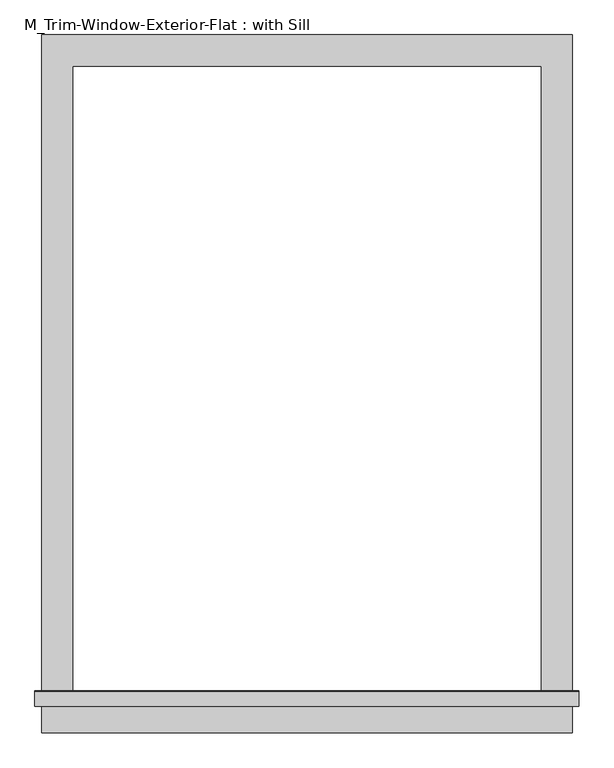
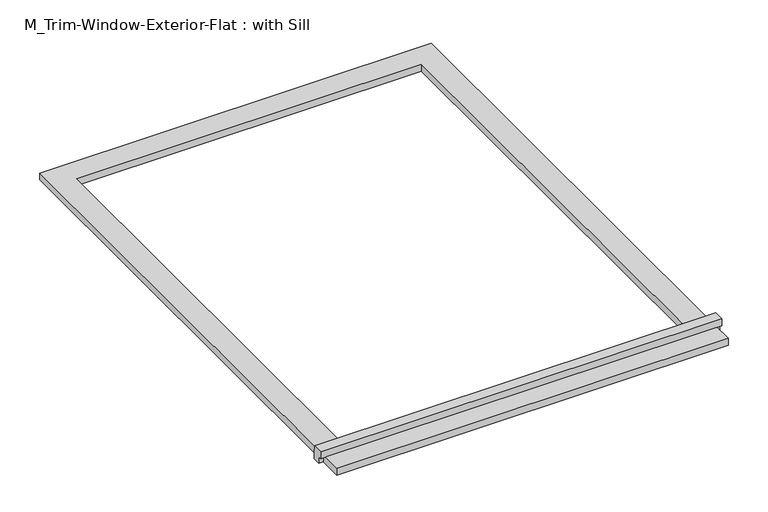
"""IFC4 building model written with IfcOpenShell, lengths in millimetres: proxy geometry, M_Trim-Window-Exterior-Flat : with Sill."""

import ifcopenshell
import ifcopenshell.guid

model = None  # the IFC model being written
_history = None  # IfcOwnerHistory: only IFC2X3 demands one
_inside = {}  # id of a spatial element -> (the spatial element, [elements in it])
_under = {}  # id of a project, library or spatial element -> (it, [spatial elements below it])
_declared = {}  # id of a project -> (the project, [libraries it declares])
_typed = {}  # id of a type object -> (the type object, [elements of that type])
_made_of = {}  # id of a material, layer set ... -> (it, [elements and type objects made of it])


def new_model(schema):
    """Start an empty IFC model of exactly this schema.

    Asked for "IFC4X3", IfcOpenShell would pick the latest addendum, in which some entities
    have other attributes; the version numbers below select the first issue.
    IFC2X3 requires an IfcOwnerHistory on every rooted entity: one is made here for all.
    """
    global model, _history
    if schema == "IFC4X3":
        model = ifcopenshell.file(schema_version=(4, 3, 0, 0))
    else:
        model = ifcopenshell.file(schema=schema)
    _inside.clear()
    _under.clear()
    _declared.clear()
    _typed.clear()
    _made_of.clear()
    _history = None
    if model.schema == "IFC2X3":
        org = make("IfcOrganization", Name="unknown")
        user = make(
            "IfcPersonAndOrganization",
            ThePerson=make("IfcPerson", FamilyName="unknown"),
            TheOrganization=org,
        )
        app = make(
            "IfcApplication",
            ApplicationDeveloper=org,
            Version="unknown",
            ApplicationFullName="unknown",
            ApplicationIdentifier="unknown",
        )
        _history = make(
            "IfcOwnerHistory",
            OwningUser=user,
            OwningApplication=app,
            ChangeAction="ADDED",
            CreationDate=0,
        )
    return model


def make(cls, **values):
    """One entity of the class cls with the attributes given. An attribute that is None is left unset."""
    return model.create_entity(
        cls, **{name: value for name, value in values.items() if value is not None}
    )


def rooted(cls, **values):
    """An entity with a GlobalId (a new one), such as an element, a storey or a relation."""
    return make(cls, GlobalId=ifcopenshell.guid.new(), OwnerHistory=_history, **values)


def si_unit(unit_type, name, prefix=None):
    """IfcSIUnit, for example si_unit("LENGTHUNIT", "METRE", prefix="MILLI")."""
    return make("IfcSIUnit", UnitType=unit_type, Prefix=prefix, Name=name)


def assignment(units):
    """IfcUnitAssignment: the units of a project."""
    return None if units is None else make("IfcUnitAssignment", Units=units)


def point(xyz):
    """IfcCartesianPoint."""
    return None if xyz is None else make("IfcCartesianPoint", Coordinates=xyz)


def direction(xyz):
    """IfcDirection."""
    return None if xyz is None else make("IfcDirection", DirectionRatios=xyz)


def frame(location, z_axis=None, x_axis=None):
    """IfcAxis2Placement3D, a coordinate frame: its origin and axes. An axis left out is left unset."""
    return make(
        "IfcAxis2Placement3D",
        Location=point(location),
        Axis=direction(z_axis),
        RefDirection=direction(x_axis),
    )


def origin():
    """The frame at (0, 0, 0) with its axes left unset."""
    return frame((0.0, 0.0, 0.0))


def origin_with_axes():
    """The frame at (0, 0, 0) with the z axis (0, 0, 1) and the x axis (1, 0, 0) written out."""
    return frame((0.0, 0.0, 0.0), z_axis=(0.0, 0.0, 1.0), x_axis=(1.0, 0.0, 0.0))


def place(relative_to, where):
    """IfcLocalPlacement: puts the frame where relative to a parent placement (None: the world)."""
    return make(
        "IfcLocalPlacement", PlacementRelTo=relative_to, RelativePlacement=where
    )


def context(
    kind, dimensions, precision=None, world=None, true_north=None, identifier=None
):
    """IfcGeometricRepresentationContext, for example the 3D "Model" context."""
    return make(
        "IfcGeometricRepresentationContext",
        ContextIdentifier=identifier,
        ContextType=kind,
        CoordinateSpaceDimension=dimensions,
        Precision=precision,
        WorldCoordinateSystem=world,
        TrueNorth=true_north,
    )


def project(units=None, contexts=None):
    """IfcProject with its units and contexts."""
    return rooted(
        "IfcProject",
        Name="project",
        RepresentationContexts=contexts,
        UnitsInContext=assignment(units),
    )


def spatial(cls, under=None, at=None, **own):
    """A site, building, storey or space (cls), placed at a placement, below another one or the project."""
    s = rooted(cls, ObjectPlacement=at, **own)
    if under is not None:
        _under.setdefault(under.id(), (under, []))[1].append(s)
    return s


def polyline(points):
    """IfcPolyline through the points."""
    return make("IfcPolyline", Points=[point(p) for p in points])


def outline(outer, holes=None, kind="AREA"):
    """IfcArbitraryClosedProfileDef: a profile drawn as a closed curve; with holes, ...WithVoids."""
    if holes is None:
        return make("IfcArbitraryClosedProfileDef", ProfileType=kind, OuterCurve=outer)
    return make(
        "IfcArbitraryProfileDefWithVoids",
        ProfileType=kind,
        OuterCurve=outer,
        InnerCurves=holes,
    )


def extrude(swept, where, along, depth):
    """IfcExtrudedAreaSolid: the profile swept, set in the frame where, extruded along a direction by depth."""
    return make(
        "IfcExtrudedAreaSolid",
        SweptArea=swept,
        Position=where,
        ExtrudedDirection=direction(along),
        Depth=depth,
    )


def shape(context_of_items, identifier, shape_type, items):
    """IfcShapeRepresentation: the items that make up one representation, for example the "Body"."""
    return make(
        "IfcShapeRepresentation",
        ContextOfItems=context_of_items,
        RepresentationIdentifier=identifier,
        RepresentationType=shape_type,
        Items=items,
    )


def source(mapping_origin, context_of_items, identifier, shape_type, items):
    """IfcRepresentationMap: a shape defined once, which mapped items show again and again."""
    return make(
        "IfcRepresentationMap",
        MappingOrigin=mapping_origin,
        MappedRepresentation=shape(context_of_items, identifier, shape_type, items),
    )


def transform(
    local_origin,
    x_axis=None,
    y_axis=None,
    z_axis=None,
    scale=None,
    scale2=None,
    scale3=None,
    uniform=True,
):
    """IfcCartesianTransformationOperator3D, or its non-uniform kind. x_axis, y_axis, z_axis: its Axis1, 2, 3."""
    if uniform:
        return make(
            "IfcCartesianTransformationOperator3D",
            Axis1=direction(x_axis),
            Axis2=direction(y_axis),
            LocalOrigin=point(local_origin),
            Scale=scale,
            Axis3=direction(z_axis),
        )
    return make(
        "IfcCartesianTransformationOperator3DnonUniform",
        Axis1=direction(x_axis),
        Axis2=direction(y_axis),
        LocalOrigin=point(local_origin),
        Scale=scale,
        Axis3=direction(z_axis),
        Scale2=scale2,
        Scale3=scale3,
    )


def mapped(mapping_source, mapping_target):
    """IfcMappedItem: shows the shape of a source again, moved by a transform."""
    return make(
        "IfcMappedItem", MappingSource=mapping_source, MappingTarget=mapping_target
    )


def made_of(thing, what):
    """Note that an element or type object is made of a material, layer set ...; save() writes the relation."""
    if what is not None:
        _made_of.setdefault(what.id(), (what, []))[1].append(thing)
    return thing


def element(
    cls,
    number,
    at=None,
    inside=None,
    cuts=None,
    type_object=None,
    material=None,
    context=None,
    identifier="Body",
    shape_type=None,
    held_by="IfcProductDefinitionShape",
    body=None,
    shapes=None,
    **own,
):
    """One element of the class cls, such as IfcWall. Its Tag is "e" and its number.

    at: its placement. inside: the storey or other place that contains it. cuts: it is an
    opening in that element (IfcRelVoidsElement). A single representation is given by context,
    identifier, shape_type and body (its items); several are given by shapes. held_by: the class
    of the entity that holds the representations. save() writes the other relations.
    """
    e = rooted(cls, Tag="e%d" % number, ObjectPlacement=at, **own)
    if body is not None:
        shapes = [shape(context, identifier, shape_type, body)]
    if shapes is not None:
        e.Representation = make(held_by, Representations=shapes)
    if inside is not None:
        _inside.setdefault(inside.id(), (inside, []))[1].append(e)
    if cuts is not None:
        rooted(
            "IfcRelVoidsElement", RelatingBuildingElement=cuts, RelatedOpeningElement=e
        )
    if type_object is not None:
        _typed.setdefault(type_object.id(), (type_object, []))[1].append(e)
    return made_of(e, material)


def aggregate(whole, parts):
    """IfcRelAggregates: a whole, such as a stair, and the parts it consists of."""
    return rooted("IfcRelAggregates", RelatingObject=whole, RelatedObjects=parts)


def save(model, path):
    """Write the relations noted so far, then the file.

    IfcRelAggregates (storeys below a building ...), IfcRelContainedInSpatialStructure (elements
    in a storey), IfcRelDefinesByType, IfcRelAssociatesMaterial and IfcRelDeclares: one each for
    every whole, place, type object, material and project.
    """
    for whole, parts in _under.values():
        aggregate(whole, parts)
    for where, things in _inside.values():
        rooted(
            "IfcRelContainedInSpatialStructure",
            RelatedElements=things,
            RelatingStructure=where,
        )
    for kind, things in _typed.values():
        rooted("IfcRelDefinesByType", RelatedObjects=things, RelatingType=kind)
    for what, things in _made_of.values():
        rooted("IfcRelAssociatesMaterial", RelatedObjects=things, RelatingMaterial=what)
    for by, libraries in _declared.values():
        rooted("IfcRelDeclares", RelatingContext=by, RelatedDefinitions=libraries)
    model.write(path)


def m_trim_window_exterior_flat_with_sill_71544b40(model_context):
    return source(origin(), model_context, "Body", "SweptSolid", [
        extrude(outline(polyline([(510.0, -1220.4323709), (510.0, -1280.4323709), (-510.0, -1280.4323709), (-510.0, -1220.4323709), (510.0, -1220.4323709)])), origin_with_axes(), (0.0, 0.0, 1.0), 19.05),
        extrude(outline(polyline([(-1230.0, 38.1), (-1202.4580645, 38.1), (-1200.0, 19.05), (-1200.0, 0.0), (-1220.4323709, 0.0), (-1220.4323709, 19.05), (-1230.0, 19.05), (-1230.0, 38.1)])), frame((-522.7, 0.0, 0.0), z_axis=(1.0, 0.0, 0.0), x_axis=(0.0, 1.0, 0.0)), (0.0, 0.0, 1.0), 1045.4),
        extrude(outline(polyline([(-510.0, 60.0), (510.0, 60.0), (510.0, -1200.0), (450.0, -1200.0), (450.0, 0.0), (-450.0, 0.0), (-450.0, -1200.0), (-510.0, -1200.0), (-510.0, 60.0)])), origin_with_axes(), (0.0, 0.0, 1.0), 19.05),
    ])


if __name__ == "__main__":
    model = new_model("IFC4")
    model_context = context("Model", 3, world=origin())
    ifc_project = project(units=[si_unit("LENGTHUNIT", "METRE", prefix="MILLI")], contexts=[model_context])
    site = spatial("IfcSite", under=ifc_project)
    building = spatial("IfcBuilding", under=site)
    placement = place(None, origin())
    m_trim_window_exterior_flat_with_sill_shape = m_trim_window_exterior_flat_with_sill_71544b40(model_context)
    element("IfcBuildingElementProxy", 1, Name="M_Trim-Window-Exterior-Flat : with Sill", ObjectType="M_Trim-Window-Exterior-Flat : with Sill", at=placement, inside=building, context=model_context, shape_type="MappedRepresentation", body=[
        mapped(m_trim_window_exterior_flat_with_sill_shape, transform((0.0, 0.0, 0.0), x_axis=(1.0, 0.0, 0.0), y_axis=(0.0, 1.0, 0.0), z_axis=(0.0, 0.0, 1.0))),
    ])
    save(model, "model.ifc")

# Revit data of these elements
# Project information
#   Название организации = "Organization Name"
#   Описание организации = "Organization Description"
#   Наименование здания = "Building Name"
#   Дата утверждения проекта = "Issue Date"
#   Статус проекта = "Project Status"
#   Заказчик = "Client Name"
#   Адрес проекта = "Enter address here\nAddress Line 2"
#   Наименование проекта = "Project Name"
#   Номер проекта = "Project Number"
# Type "M_Trim-Window-Exterior-Flat : with Sill"
#   Trim Width = 60 mm
#   Trim Thickness_Picture Frame = 30 mm
#   Trim Thickness_with Sill = 19.05 mm
#   Sill Thickness = 30 mm
#   Opening Width [instance default] = 600 mm
#   Opening Height [instance default] = 900 mm
#   Default Elevation = 1200 mm
#   Sill = yes
#   Picture Frame = no
#   Trim Material [instance default] = none
# Element 1 (IfcBuildingElementProxy, "M_Trim-Window-Exterior-Flat : with Sill")
#   Opening Width = 900 mm
#   Opening Height = 1200 mm
#   Trim Material = Clad - White
#   Materials on its faces: "Clad - White"
# Materials
#   "Clad - White": class "Wood", colour RGB 245 245 243, transparency 0, Cost = 0
